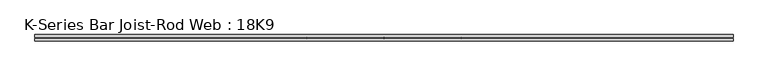
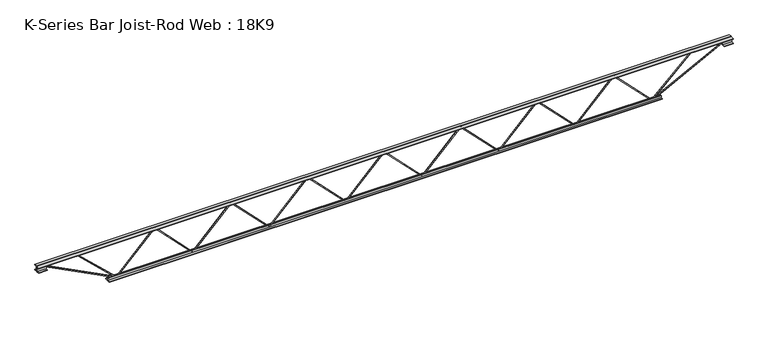
"""IFC4 building model written with IfcOpenShell, lengths in millimetres: beam geometry, K-Series Bar Joist-Rod Web : 18K9."""

from ifc_helpers import new_model, si_unit, frame, origin, place, context, project, spatial, polyline, outline, extrude, source, transform, mapped, element, save


def k_series_bar_joist_rod_web_18k9_f4150f3c(model_context):
    return source(origin(), model_context, "Body", "SweptSolid", [
        extrude(outline(polyline([(-217.4875, 1321.2535714), (-227.0125, 1321.2535714), (-227.0125, 1326.4344703), (217.4875, 1760.5023274), (217.4875, 1762.8405297), (-227.0125, 2196.9083869), (-227.0125, 2202.0892857), (-217.4875, 2202.0892857), (-217.4875, 2200.9201846), (227.0125, 1766.8523274), (227.0125, 1756.4905297), (-217.4875, 1322.4226726), (-217.4875, 1321.2535714)])), frame((0.0, -4.7625, 0.0), z_axis=(0.0, 1.0, 0.0), x_axis=(0.0, 0.0, 1.0)), (0.0, 0.0, 1.0), 9.525),
        extrude(outline(polyline([(-217.4875, 440.4178571), (-227.0125, 440.4178571), (-227.0125, 445.598756), (217.4875, 879.6666131), (217.4875, 882.0048154), (-227.0125, 1316.0726726), (-227.0125, 1321.2535714), (-217.4875, 1321.2535714), (-217.4875, 1320.0844703), (227.0125, 886.0166131), (227.0125, 875.6548154), (-217.4875, 441.5869583), (-217.4875, 440.4178571)])), frame((0.0, -4.7625, 0.0), z_axis=(0.0, 1.0, 0.0), x_axis=(0.0, 0.0, 1.0)), (0.0, 0.0, 1.0), 9.525),
        extrude(outline(polyline([(-217.4875, -440.4178571), (-227.0125, -440.4178571), (-227.0125, -435.2369583), (217.4875, -1.1691011), (217.4875, 1.1691011), (-227.0125, 435.2369583), (-227.0125, 440.4178571), (-217.4875, 440.4178571), (-217.4875, 439.248756), (227.0125, 5.1808989), (227.0125, -5.1808989), (-217.4875, -439.248756), (-217.4875, -440.4178571)])), frame((0.0, -4.7625, 0.0), z_axis=(0.0, 1.0, 0.0), x_axis=(0.0, 0.0, 1.0)), (0.0, 0.0, 1.0), 9.525),
        extrude(outline(polyline([(-217.4875, -1321.2535714), (-227.0125, -1321.2535714), (-227.0125, -1316.0726726), (217.4875, -882.0048154), (217.4875, -879.6666131), (-227.0125, -445.598756), (-227.0125, -440.4178571), (-217.4875, -440.4178571), (-217.4875, -441.5869583), (227.0125, -875.6548154), (227.0125, -886.0166131), (-217.4875, -1320.0844703), (-217.4875, -1321.2535714)])), frame((0.0, -4.7625, 0.0), z_axis=(0.0, 1.0, 0.0), x_axis=(0.0, 0.0, 1.0)), (0.0, 0.0, 1.0), 9.525),
        extrude(outline(polyline([(-217.4875, -2202.0892857), (-227.0125, -2202.0892857), (-227.0125, -2196.9083869), (217.4875, -1762.8405297), (217.4875, -1760.5023274), (-227.0125, -1326.4344703), (-227.0125, -1321.2535714), (-217.4875, -1321.2535714), (-217.4875, -1322.4226726), (227.0125, -1756.4905297), (227.0125, -1766.8523274), (-217.4875, -2200.9201846), (-217.4875, -2202.0892857)])), frame((0.0, -4.7625, 0.0), z_axis=(0.0, 1.0, 0.0), x_axis=(0.0, 0.0, 1.0)), (0.0, 0.0, 1.0), 9.525),
        extrude(outline(polyline([(-217.4875, 2202.0892857), (-227.0125, 2202.0892857), (-227.0125, 2207.2701846), (217.4875, 2641.3380417), (217.4875, 2643.676244), (-227.0125, 3077.7441011), (-227.0125, 3082.925), (-217.4875, 3082.925), (-217.4875, 3081.7558989), (227.0125, 2647.6880417), (227.0125, 2637.326244), (-217.4875, 2203.2583869), (-217.4875, 2202.0892857)])), frame((0.0, -4.7625, 0.0), z_axis=(0.0, 1.0, 0.0), x_axis=(0.0, 0.0, 1.0)), (0.0, 0.0, 1.0), 9.525),
        extrude(outline(polyline([(-217.4875, -3082.925), (-227.0125, -3082.925), (-227.0125, -3077.7441011), (217.4875, -2643.676244), (217.4875, -2641.3380417), (-227.0125, -2207.2701846), (-227.0125, -2202.0892857), (-217.4875, -2202.0892857), (-217.4875, -2203.2583869), (227.0125, -2637.326244), (227.0125, -2647.6880417), (-217.4875, -3081.7558989), (-217.4875, -3082.925)])), frame((0.0, -4.7625, 0.0), z_axis=(0.0, 1.0, 0.0), x_axis=(0.0, 0.0, 1.0)), (0.0, 0.0, 1.0), 9.525),
        extrude(outline(polyline([(4.7625, 228.6), (36.5125, 228.6), (36.5125, 222.25), (11.1125, 222.25), (11.1125, 196.85), (4.7625, 196.85), (4.7625, 228.6)])), frame((-3997.325, 0.0, 0.0), z_axis=(1.0, 0.0, 0.0), x_axis=(0.0, 1.0, 0.0)), (0.0, 0.0, 1.0), 7994.65),
        extrude(outline(polyline([(-4.7625, 228.6), (-4.7625, 196.85), (-11.1125, 196.85), (-11.1125, 222.25), (-36.5125, 222.25), (-36.5125, 228.6), (-4.7625, 228.6)])), frame((-3997.325, 0.0, 0.0), z_axis=(1.0, 0.0, 0.0), x_axis=(0.0, 1.0, 0.0)), (0.0, 0.0, 1.0), 7994.65),
        extrude(outline(polyline([(-4.7625, 165.1), (-36.5125, 165.1), (-36.5125, 171.45), (-11.1125, 171.45), (-11.1125, 196.85), (-4.7625, 196.85), (-4.7625, 165.1)])), frame((-3997.325, 0.0, 0.0), z_axis=(1.0, 0.0, 0.0), x_axis=(0.0, 1.0, 0.0)), (0.0, 0.0, 1.0), 101.6),
        extrude(outline(polyline([(36.5125, 165.1), (4.7625, 165.1), (4.7625, 196.85), (11.1125, 196.85), (11.1125, 171.45), (36.5125, 171.45), (36.5125, 165.1)])), frame((-3997.325, 0.0, 0.0), z_axis=(1.0, 0.0, 0.0), x_axis=(0.0, 1.0, 0.0)), (0.0, 0.0, 1.0), 101.6),
        extrude(outline(polyline([(4.7625, 165.1), (4.7625, 196.85), (11.1125, 196.85), (11.1125, 171.45), (36.5125, 171.45), (36.5125, 165.1), (4.7625, 165.1)])), frame((3895.725, 0.0, 0.0), z_axis=(1.0, 0.0, 0.0), x_axis=(0.0, 1.0, 0.0)), (0.0, 0.0, 1.0), 101.6),
        extrude(outline(polyline([(-4.7625, 165.1), (-36.5125, 165.1), (-36.5125, 171.45), (-11.1125, 171.45), (-11.1125, 196.85), (-4.7625, 196.85), (-4.7625, 165.1)])), frame((3895.725, 0.0, 0.0), z_axis=(1.0, 0.0, 0.0), x_axis=(0.0, 1.0, 0.0)), (0.0, 0.0, 1.0), 101.6),
        extrude(outline(polyline([(4.7625, -228.6), (4.7625, -196.85), (11.1125, -196.85), (11.1125, -222.25), (36.5125, -222.25), (36.5125, -228.6), (4.7625, -228.6)])), frame((-3184.525, 0.0, 0.0), z_axis=(1.0, 0.0, 0.0), x_axis=(0.0, 1.0, 0.0)), (0.0, 0.0, 1.0), 6369.05),
        extrude(outline(polyline([(-4.7625, -228.6), (-36.5125, -228.6), (-36.5125, -222.25), (-11.1125, -222.25), (-11.1125, -196.85), (-4.7625, -196.85), (-4.7625, -228.6)])), frame((-3184.525, 0.0, 0.0), z_axis=(1.0, 0.0, 0.0), x_axis=(0.0, 1.0, 0.0)), (0.0, 0.0, 1.0), 6369.05),
        extrude(outline(polyline([(0.0, -9.525), (0.0, 0.0), (914.4881902, 0.0), (914.4881902, -9.525), (0.0, -9.525)])), frame((-3897.907602, 4.7625, 192.6170749), z_axis=(0.4582891331947272, 0.0, 0.888803167408637), x_axis=(0.888803167408637, 0.0, -0.4582891331947272)), (0.0, 0.0, 1.0), 9.525),
        extrude(outline(polyline([(0.0, -9.525), (0.0, 0.0), (607.9578102, 0.0), (607.9578102, -9.525), (0.0, -9.525)])), frame((-3526.6259201, 4.7625, 193.3999414), z_axis=(0.6893570458690655, 0.0, 0.7244217440901916), x_axis=(0.7244217440901916, 0.0, -0.6893570458690655)), (0.0, 0.0, 1.0), 9.525),
        extrude(outline(polyline([(0.0, -9.525), (0.0, 0.0), (914.4881902, 0.0), (914.4881902, -9.525), (0.0, -9.525)])), frame((3897.907602, -4.7625, 192.6170749), z_axis=(-0.45828913319471537, 0.0, 0.8888031674086432), x_axis=(-0.8888031674086432, 0.0, -0.45828913319471537)), (0.0, 0.0, 1.0), 9.525),
        extrude(outline(polyline([(0.0, -9.525), (0.0, 0.0), (607.9578102, 0.0), (607.9578102, -9.525), (0.0, -9.525)])), frame((3526.6259201, -4.7625, 193.3999414), z_axis=(-0.6893570458690618, 0.0, 0.7244217440901952), x_axis=(-0.7244217440901952, 0.0, -0.6893570458690618)), (0.0, 0.0, 1.0), 9.525),
    ])


if __name__ == "__main__":
    model = new_model("IFC4")
    model_context = context("Model", 3, world=origin())
    ifc_project = project(units=[si_unit("LENGTHUNIT", "METRE", prefix="MILLI")], contexts=[model_context])
    site = spatial("IfcSite", under=ifc_project)
    building = spatial("IfcBuilding", under=site)
    placement = place(None, origin())
    k_series_bar_joist_rod_web_18k9_shape = k_series_bar_joist_rod_web_18k9_f4150f3c(model_context)
    element("IfcBeam", 1, ObjectType="K-Series Bar Joist-Rod Web : 18K9", at=placement, inside=building, context=model_context, shape_type="MappedRepresentation", body=[
        mapped(k_series_bar_joist_rod_web_18k9_shape, transform((0.0, 0.0, 0.0), x_axis=(1.0, 0.0, 0.0), y_axis=(0.0, 1.0, 0.0), z_axis=(0.0, 0.0, 1.0))),
    ])
    save(model, "model.ifc")

# Revit data of these elements
# Type "K-Series Bar Joist-Rod Web : 18K9"
#   Assembly Code = "B1010350"
#   Wt = 10.2
#   Web Thickness = 0' - 0 3/8"
#   Start Offset [instance default] = 0' - 0"
#   Start Extension [instance default] = 0' - 0"
#   Seat Length = 0' - 4"
#   Seat Depth = 0' - 2 1/2"
#   PanelArrayLength [instance default] = 18' - 0"
#   Panel [instance default] = 3' - 0"
#   End Offset [instance default] = 0' - 0"
#   End Extension [instance default] = 0' - 0"
#   End Panel = 3' - 0"
#   Cord Leg = 0' - 1 1/4"
#   Chord Thickness = 0' - 0 1/4"
#   Length [instance default] = 24' - 0"
#   Depth = 1' - 6"
#   PanelArrayNum [instance default] = 6
#   Structural Material = none
# Element 1 (IfcBeam, "K-Series Bar Joist-Rod Web : 18K9")
#   PanelArrayLength = 20' - 2 3/4"
#   Panel = 2' - 10.67857"
#   PanelArrayNum = 7
